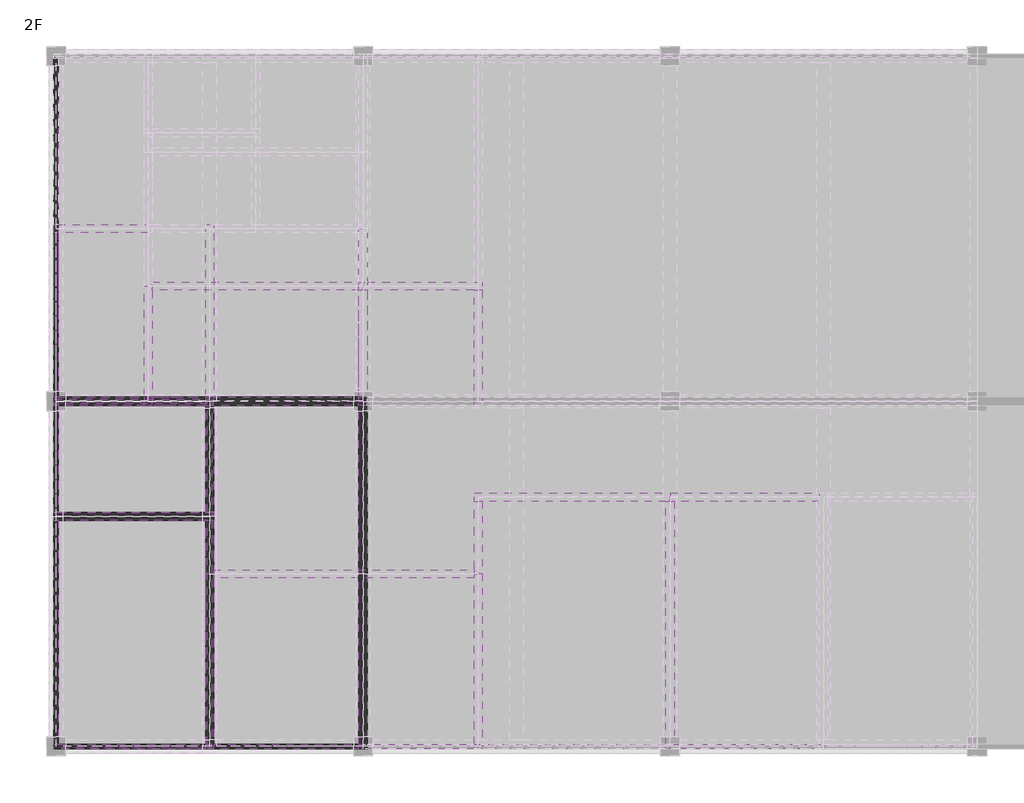
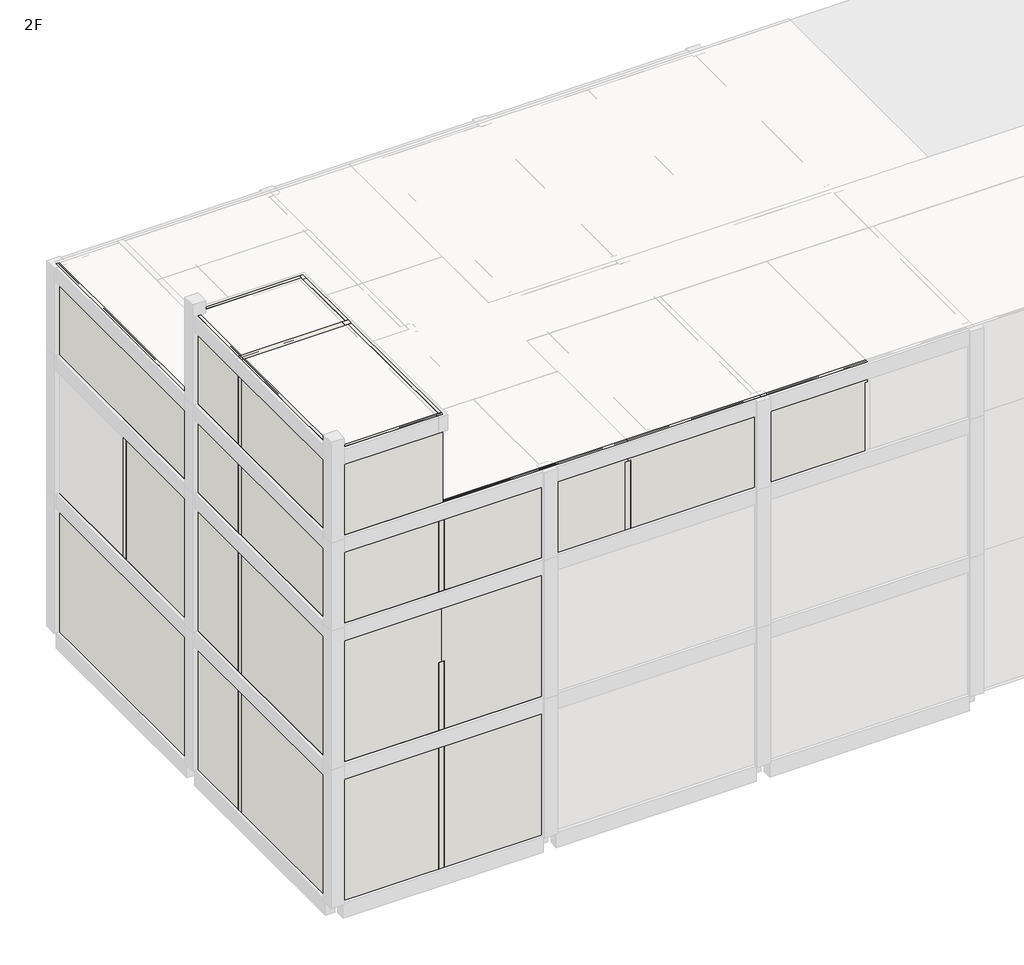
# One storey, part 1 of 7: 56 walls.
# Revit data of these elements (continued)
# Materials (continued)
#   "A04AK069-00002_Reinforced Concrete Block_THK 100-200mm": class "Concrete", colour RGB 180 180 180, transparency 0, Description = "Conc. Block", W00) Work Master Code = "A04AK069-00002", W01) Work Master_Lv1 = "Finishing Work", W02) Work Master_Lv2 = "Masonry Work", W03) Work Master_Spec.1 = "Reinforced Concrete Block", W04) Work Master_Spec.2 = "w/ All Reinf.(Lath, Steel Tie, Anchor Bar, Mortar, ETC.), Filler, Sealant, Lintel/Sill for Opening, ETC.", W05) Work Master_Spec.3 = "100mm<THK≤200mm", Cost = 0
#   "Default Wall": class "Miscellaneous", colour RGB 80 80 80, transparency 0
# Room at (79959.652, 167173.861) mm, phase "New Construction", upper offset 2700 mm, lower offset 0 mm
#   Department = "AR"
#   Base Finish = "WK3"
#   Ceiling Finish = "CL3"
#   Wall Finish = "IW5"
#   Floor Finish = "FL2"
#   Number = "4.5"
#   Name = "Office-1"
#   Interior Finish = "IW5..N/A..N/A,,WK3..N/A,,FL2..N/A,,CL3..N/A"
#   Exterior Finish = "RF1..N/A,,EW2..N/A..N/A"
# Room at (84959.652, 167173.861) mm, phase "New Construction", upper offset 3500 mm, lower offset 0 mm
#   Department = "FF"
#   Base Finish = "WK1"
#   Ceiling Finish = ""
#   Wall Finish = "IW5"
#   Floor Finish = "FL1"
#   Number = "4.6"
#   Name = "Fire Gas Room"
#   Interior Finish = "IW5..N/A..N/A,,WK1..N/A,,FL1..N/A,,N/A..N/A"
#   Exterior Finish = "RF1..N/A,,EW2..N/A..N/A"
# Room at (78709.652, 174423.861) mm, phase "New Construction", upper offset 2700 mm, lower offset 0 mm
#   Department = "AR"
#   Base Finish = "WK3"
#   Ceiling Finish = "CL3"
#   Wall Finish = "IW5"
#   Floor Finish = "FL2"
#   Number = "4.7"
#   Name = "Document Room"
#   Interior Finish = "IW5..N/A..N/A,,WK3..N/A,,FL2..N/A,,CL3..N/A"
#   Exterior Finish = "RF1..N/A,,N/A..N/A..N/A"
# Room at (58959.652, 167173.861) mm, phase "New Construction", upper offset 2700 mm, lower offset 0 mm
#   Department = "AR"
#   Base Finish = "WK3"
#   Ceiling Finish = "CL3"
#   Wall Finish = "IW5"
#   Floor Finish = "FL2"
#   Number = "4.8"
#   Name = "Storage"
#   Interior Finish = "IW5..N/A..N/A,,WK3..N/A,,FL2..N/A,,CL3..N/A"
#   Exterior Finish = "RF1..N/A,,EW1..N/A..N/A"
# Room at (52959.652, 166173.861) mm, phase "New Construction", upper offset 2700 mm, lower offset 0 mm
#   Department = "AR"
#   Base Finish = "WK3"
#   Ceiling Finish = "CL3"
#   Wall Finish = "IW5"
#   Floor Finish = "FL2"
#   Number = "4.9"
#   Name = "Break Room"
#   Interior Finish = "IW5..N/A..N/A,,WK3..N/A,,FL2..N/A,,CL3..N/A"
#   Exterior Finish = "RF1..N/A,,EW2..N/A..N/A"
# Room at (50659.652, 177673.861) mm, phase "New Construction", upper offset 2700 mm, lower offset 0 mm
#   Department = "AR"
#   Base Finish = ""
#   Ceiling Finish = "CL4"
#   Wall Finish = "IW3"
#   Floor Finish = "FL3"
#   Number = "4.10"
#   Name = "Toilet"
#   Interior Finish = "IW3..N/A..N/A,,N/A..N/A,,FL3..N/A,,CL4..N/A"
#   Exterior Finish = "RF1..N/A,,N/A..N/A..N/A"
# Room at (50659.652, 180673.861) mm, phase "New Construction", upper offset 2700 mm, lower offset 0 mm
#   Department = "AR"
#   Base Finish = ""
#   Ceiling Finish = "CL4"
#   Wall Finish = "IW3"
#   Floor Finish = "FL3"
#   Number = "4.11"
#   Name = "Shower"
#   Interior Finish = "IW3..N/A..N/A,,N/A..N/A,,FL3..N/A,,CL4..N/A"
#   Exterior Finish = "RF1..N/A,,EW2..N/A..N/A"
# Room at (61459.652, 177423.861) mm, phase "New Construction", upper offset 5500 mm, lower offset 0 mm
#   Department = "CI"
#   Base Finish = "WK1"
#   Ceiling Finish = "CL1"
#   Wall Finish = "IW5"
#   Floor Finish = "FL1"
#   Number = "2.0"
#   Name = "Electrical Room-1"
#   Interior Finish = "IW5..N/A..N/A,,WK1..N/A,,FL1..N/A,,CL1..N/A"
#   Exterior Finish = "N/A..N/A,,EW1..EW2..N/A"
# Room at (70459.652, 168423.861) mm, phase "New Construction", upper offset 5500 mm, lower offset 0 mm
#   Department = "EL"
#   Base Finish = "WK1"
#   Ceiling Finish = "CL1"
#   Wall Finish = "IW5"
#   Floor Finish = "FL1"
#   Number = "2.1"
#   Name = "Electrical Room-2"
#   Interior Finish = "IW5..N/A..N/A,,WK1..N/A,,FL1..N/A,,CL1..N/A"
#   Exterior Finish = "N/A..N/A,,EW1..EW2..N/A"
# Room at (82459.652, 177423.861) mm, phase "New Construction", upper offset 5500 mm, lower offset 0 mm
#   Department = "AR"
#   Base Finish = "WK1"
#   Ceiling Finish = "CL1"
#   Wall Finish = "IW5"
#   Floor Finish = "FL1"
#   Number = "2.2"
#   Name = "Electrical Room (GIS)"
#   Interior Finish = "IW5..N/A..N/A,,WK1..N/A,,FL1..N/A,,CL1..N/A"
#   Exterior Finish = "N/A..N/A,,EW1..EW2..N/A"
# Room at (51459.652, 168423.861) mm, phase "New Construction", upper offset 2700 mm, lower offset 0 mm
#   Department = "AR"
#   Base Finish = "WK3"
#   Ceiling Finish = "CL3"
#   Wall Finish = "IW5"
#   Floor Finish = "FL2"
#   Number = "2.3"
#   Name = "Lobby"
#   Interior Finish = "IW5..N/A..N/A,,WK3..N/A,,FL2..N/A,,CL3..N/A"
#   Exterior Finish = "N/A..N/A,,EW2..N/A..N/A"
# Room at (47459.652, 171423.861) mm, phase "New Construction", upper offset 5500 mm, lower offset 0 mm
#   Department = "PATHV2"
#   Base Finish = ""
#   Ceiling Finish = ""
#   Wall Finish = ""
#   Floor Finish = ""
#   Number = "2.4"
#   Name = "Elevator"
#   Interior Finish = "N/A..N/A..N/A,,N/A..N/A,,N/A..N/A,,N/A..N/A"
#   Exterior Finish = "N/A..N/A,,EW2..N/A..N/A"
# Room at (47459.652, 166923.861) mm, phase "New Construction", upper offset 5500 mm, lower offset 0 mm
#   Department = "PATHV1"
#   Base Finish = "WK3"
#   Ceiling Finish = "CL1"
#   Wall Finish = "IW5"
#   Floor Finish = "FL2"
#   Number = "2.5"
#   Name = "Staircase"
#   Interior Finish = "IW5..N/A..N/A,,WK3..N/A,,FL2..N/A,,CL1..N/A"
#   Exterior Finish = "N/A..N/A,,EW2..N/A..N/A"
# Room at (65459.652, 177423.861) mm, phase "New Construction", upper offset 3400 mm, lower offset 0 mm
#   Department = "CI"
#   Base Finish = ""
#   Ceiling Finish = "CL3"
#   Wall Finish = "IW5"
#   Floor Finish = "FL5"
#   Number = "3.0"
#   Name = "Central Control Room"
#   Interior Finish = "IW5..N/A..N/A,,N/A..N/A,,FL5..N/A,,CL3..N/A"
#   Exterior Finish = "N/A..N/A,,EW1..N/A..N/A"
# Room at (65459.652, 168423.861) mm, phase "New Construction", upper offset 3000 mm, lower offset 0 mm
#   Department = "CI"
#   Base Finish = ""
#   Ceiling Finish = "CL3"
#   Wall Finish = "IW5"
#   Floor Finish = "FL5"
#   Number = "3.1"
#   Name = "Electronic Room"
#   Interior Finish = "IW5..N/A..N/A,,N/A..N/A,,FL5..N/A,,CL3..N/A"
#   Exterior Finish = "N/A..N/A,,EW1..N/A..N/A"
# Room at (80959.652, 180173.861) mm, phase "New Construction", upper offset 2700 mm, lower offset 0 mm
#   Department = "AR"
#   Base Finish = ""
#   Ceiling Finish = "CL3"
#   Wall Finish = "IW5"
#   Floor Finish = "FL5"
#   Number = "3.2"
#   Name = "Computer Room"
#   Interior Finish = "IW5..N/A..N/A,,N/A..N/A,,FL5..N/A,,CL3..N/A"
#   Exterior Finish = "N/A..N/A,,EW2..N/A..N/A"
# Room at (82459.652, 168423.861) mm, phase "New Construction", upper offset 5500 mm, lower offset 0 mm
#   Department = "EL"
#   Base Finish = ""
#   Ceiling Finish = "CL3"
#   Wall Finish = "IW5"
#   Floor Finish = "FL5"
#   Number = "3.3"
#   Name = "Electrical Room -3"
#   Interior Finish = "IW5..N/A..N/A,,N/A..N/A,,FL5,,CL3..N/A"
#   Exterior Finish = "N/A..N/A,,EW2..N/A..N/A"
# Room at (80959.652, 174673.861) mm, phase "New Construction", upper offset 2700 mm, lower offset 0 mm
#   Department = "CI"
#   Base Finish = ""
#   Ceiling Finish = "CL3"
#   Wall Finish = "IW5"
#   Floor Finish = "FL5"
#   Number = "3.4"
#   Name = "Communication Room"
#   Interior Finish = "IW5..N/A..N/A,,N/A..N/A,,FL5..N/A,,CL3..N/A"
#   Exterior Finish = "N/A..N/A,,N/A..N/A..N/A"
# Room at (46659.652, 179673.861) mm, phase "New Construction", upper offset 5500 mm, lower offset 0 mm
#   Department = "PATHV3"
#   Base Finish = ""
#   Ceiling Finish = ""
#   Wall Finish = ""
#   Floor Finish = ""
#   Number = "3.5"
#   Name = "Duct Shaft"
#   Interior Finish = "N/A..N/A..N/A,,N/A..N/A,,N/A..N/A,,N/A..N/A"
#   Exterior Finish = "N/A..N/A,,EW2..N/A..N/A"
# Room at (47459.652, 175173.861) mm, phase "New Construction", upper offset 2700 mm, lower offset 0 mm
#   Department = "AR"
#   Base Finish = ""
#   Ceiling Finish = "CL4"
#   Wall Finish = "IW3"
#   Floor Finish = "FL3"
#   Number = "3.6"
#   Name = "Toilet (M)"
#   Interior Finish = "IW3..N/A..N/A,,N/A..N/A,,FL3..N/A,,CL4..N/A"
#   Exterior Finish = "N/A..N/A,,EW2..N/A..N/A"
# Room at (52059.652, 179673.861) mm, phase "New Construction", upper offset 2700 mm, lower offset 0 mm
#   Department = "AR"
#   Base Finish = ""
#   Ceiling Finish = "CL4"
#   Wall Finish = "IW3"
#   Floor Finish = "FL3"
#   Number = "3.7"
#   Name = "Toilet"
#   Interior Finish = "IW3..N/A..N/A,,N/A..N/A,,FL3..N/A,,CL4..N/A"
#   Exterior Finish = "N/A..N/A,,EW2..N/A..N/A"
# Room at (49259.652, 180923.861) mm, phase "New Construction", upper offset 2700 mm, lower offset 0 mm
#   Department = "AR"
#   Base Finish = ""
#   Ceiling Finish = "CL4"
#   Wall Finish = "IW3"
#   Floor Finish = "FL3"
#   Number = "3.8"
#   Name = "Shower"
#   Interior Finish = "IW3..N/A..N/A,,N/A..N/A,,FL3..N/A,,CL4..N/A"
#   Exterior Finish = "N/A..N/A,,EW2..N/A..N/A"
# Room at (49259.652, 178673.861) mm, phase "New Construction", upper offset 2700 mm, lower offset 0 mm
#   Department = "AR"
#   Base Finish = "WK3"
#   Ceiling Finish = "CL3"
#   Wall Finish = "IW5"
#   Floor Finish = "FL2"
#   Number = "3.9"
#   Name = "Locker(F)"
#   Interior Finish = "IW5..N/A..N/A,,WK3..N/A,,FL2..N/A,,CL3..N/A"
#   Exterior Finish = "N/A..N/A,,N/A..N/A..N/A"
# Room at (47459.652, 171423.861) mm, phase "New Construction", upper offset 5500 mm, lower offset 0 mm
#   Department = "PATHV2"
#   Base Finish = ""
#   Ceiling Finish = ""
#   Wall Finish = ""
#   Floor Finish = ""
#   Number = "3.10"
#   Name = "Elevator"
#   Interior Finish = "N/A..N/A..N/A,,N/A..N/A,,N/A..N/A,,N/A..N/A"
#   Exterior Finish = "N/A..N/A,,EW2..N/A..N/A"
# Room at (47459.652, 166923.861) mm, phase "New Construction", upper offset 2700 mm, lower offset 0 mm
#   Department = "PATHV1"
#   Base Finish = "WK3"
#   Ceiling Finish = "CL1"
#   Wall Finish = "IW5"
#   Floor Finish = "FL2"
#   Number = "3.11"
#   Name = "Staircase"
#   Interior Finish = "IW5..N/A..N/A,,WK3..N/A,,FL2..N/A,,CL1..N/A"
#   Exterior Finish = "N/A..N/A,,EW2..N/A..N/A"
# Room at (82459.652, 177423.861) mm, phase "New Construction", upper offset 2700 mm, lower offset 0 mm
#   Department = "AR"
#   Base Finish = "WK3"
#   Ceiling Finish = "CL3"
#   Wall Finish = "IW5"
#   Floor Finish = "FL2"
#   Number = "3.12"
#   Name = "Corridor"
#   Interior Finish = "IW5..N/A..N/A,,WK3..N/A,,FL2..N/A,,CL3..N/A"
#   Exterior Finish = "N/A..N/A,,EW2..N/A..N/A"
# Room at (51459.652, 170673.861) mm, phase "New Construction", upper offset 2700 mm, lower offset 0 mm
#   Department = "AR"
#   Base Finish = "WK3"
#   Ceiling Finish = "CL3"
#   Wall Finish = "IW5"
#   Floor Finish = "FL2"
#   Number = "3.13"
#   Name = "Corridor"
#   Interior Finish = "IW5..N/A..N/A,,WK3..N/A,,FL2..N/A,,CL3..N/A"
#   Exterior Finish = "N/A..N/A,,EW2..N/A..N/A"
# Room at (63459.652, 167173.861) mm, phase "New Construction", upper offset 2700 mm, lower offset 0 mm
#   Department = "AR"
#   Base Finish = "WK3"
#   Ceiling Finish = "CL3"
#   Wall Finish = "IW5"
#   Floor Finish = "FL2"
#   Number = "4.0"
#   Name = "Manager Office-1"
#   Interior Finish = "IW5..N/A..N/A,,WK3..N/A,,FL2..N/A,,CL3..N/A"
#   Exterior Finish = "RF1..N/A,,EW1..N/A..N/A"
# Room at (67459.652, 167173.861) mm, phase "New Construction", upper offset 2700 mm, lower offset 0 mm
#   Department = "AR"
#   Base Finish = "WK3"
#   Ceiling Finish = "CL3"
#   Wall Finish = "IW5"
#   Floor Finish = "FL2"
#   Number = "4.1"
#   Name = "Manager Office-2"
#   Interior Finish = "IW5..N/A..N/A,,WK3..N/A,,FL2..N/A,,CL3..N/A"
#   Exterior Finish = "RF1..N/A,,EW1..N/A..N/A"
# Room at (78709.652, 178923.861) mm, phase "New Construction", upper offset 2700 mm, lower offset 0 mm
#   Department = "AR"
#   Base Finish = "WK3"
#   Ceiling Finish = "CL3"
#   Wall Finish = "IW5"
#   Floor Finish = "FL2"
#   Number = "4.2"
#   Name = "Meeting Room-1"
#   Interior Finish = "IW5..N/A..N/A,,WK3..N/A,,FL2..N/A,,CL3..N/A"
#   Exterior Finish = "RF1..N/A,,EW1..EW2..N/A"
# Room at (73459.652, 167173.861) mm, phase "New Construction", upper offset 2700 mm, lower offset 0 mm
#   Department = "AR"
#   Base Finish = "WK3"
#   Ceiling Finish = "CL3"
#   Wall Finish = "IW5"
#   Floor Finish = "FL2"
#   Number = "4.3"
#   Name = "Meeting Room-2"
#   Interior Finish = "IW5..N/A..N/A,,WK3..N/A,,FL2..N/A,,CL3..N/A"
#   Exterior Finish = "RF1..N/A,,EW1..N/A..N/A"
# Room at (64709.652, 177423.861) mm, phase "New Construction", upper offset 2700 mm, lower offset 0 mm
#   Department = "HV"
#   Base Finish = "WK3"
#   Ceiling Finish = "CL3"
#   Wall Finish = "IW5"
#   Floor Finish = "FL2"
#   Number = "4.4"
#   Name = "Open Office"
#   Interior Finish = "IW5..N/A..N/A,,WK3..N/A,,FL2..N/A,,CL3..N/A"
#   Exterior Finish = "RF1..N/A,,EW1..N/A..N/A"
# Room at (54959.652, 178923.861) mm, phase "New Construction", upper offset 2700 mm, lower offset 0 mm
#   Department = "AR"
#   Base Finish = "WK3"
#   Ceiling Finish = "CL3"
#   Wall Finish = "IW5"
#   Floor Finish = "FL2"
#   Number = "4.12"
#   Name = "Locker(M)"
#   Interior Finish = "IW5..N/A..N/A,,WK3..N/A,,FL2..N/A,,CL3..N/A"
#   Exterior Finish = "RF1..N/A,,EW1..N/A..N/A"
# Room at (50659.652, 174423.861) mm, phase "New Construction", upper offset 2700 mm, lower offset 0 mm
#   Department = "AR"
#   Base Finish = ""
#   Ceiling Finish = "CL4"
#   Wall Finish = "IW3"
#   Floor Finish = "FL3"
#   Number = "4.13"
#   Name = "Toilet(F)"
#   Interior Finish = "IW3..N/A..N/A,,N/A..N/A,,FL3..N/A,,CL4..N/A"
#   Exterior Finish = "RF1..N/A,,N/A..N/A..N/A"
# Room at (46659.652, 177423.861) mm, phase "New Construction", upper offset 3500 mm, lower offset 0 mm
#   Department = "PATHV3"
#   Base Finish = ""
#   Ceiling Finish = ""
#   Wall Finish = ""
#   Floor Finish = ""
#   Number = "4.14"
#   Name = "Duct Shaft"
#   Interior Finish = "N/A..N/A..N/A,,N/A..N/A,,N/A..N/A,,N/A..N/A"
#   Exterior Finish = "RF1..N/A,,EW2..N/A..N/A"
# Room at (47459.652, 171423.861) mm, phase "New Construction", upper offset 3500 mm, lower offset 0 mm
#   Department = "PATHV2"
#   Base Finish = ""
#   Ceiling Finish = ""
#   Wall Finish = ""
#   Floor Finish = ""
#   Number = "4.15"
#   Name = "Elevator"
#   Interior Finish = "N/A..N/A..N/A,,N/A..N/A,,N/A..N/A,,N/A..N/A"
#   Exterior Finish = "N/A..N/A,,EW2..N/A..N/A"
# Room at (47459.652, 166923.861) mm, phase "New Construction", upper offset 3500 mm, lower offset 0 mm
#   Department = "PATHV1"
#   Base Finish = ""
#   Ceiling Finish = "CL1"
#   Wall Finish = "IW5"
#   Floor Finish = "FL2"
#   Number = "4.16"
#   Name = "Staircase"
#   Interior Finish = "IW5..N/A..N/A,,N/A..N/A,,FL2..N/A,,CL1..N/A"
#   Exterior Finish = "N/A..N/A,,EW2..N/A..N/A"
# Room at (61397.694, 171673.861) mm, phase "New Construction", upper offset 2700 mm, lower offset 0 mm
#   Department = "AR"
#   Base Finish = "WK3"
#   Ceiling Finish = "CL3"
#   Wall Finish = "IW5"
#   Floor Finish = "FL2"
#   Number = "4.17"
#   Name = "Corridor"
#   Interior Finish = "IW5..N/A..N/A,,WK3..N/A,,FL2..N/A,,CL3..N/A"
#   Exterior Finish = "RF1..N/A,,EW2..N/A..N/A"
# Room at (47459.652, 171423.861) mm, phase "New Construction", upper offset 3500 mm, lower offset 0 mm
#   Department = "PATHV2"
#   Base Finish = ""
#   Ceiling Finish = ""
#   Wall Finish = ""
#   Floor Finish = ""
#   Number = "5.0"
#   Name = "Elevator"
#   Interior Finish = "N/A..N/A..N/A,,N/A..N/A,,N/A..N/A,,N/A..N/A"
#   Exterior Finish = "RF1..N/A,,EW2..EW1..N/A"
# Room at (47459.652, 166923.861) mm, phase "New Construction", upper offset 3500 mm, lower offset 0 mm
#   Department = "PATHV1"
#   Base Finish = "WK3"
#   Ceiling Finish = "CL1"
#   Wall Finish = "IW5"
#   Floor Finish = "FL2"
#   Number = "5.1"
#   Name = "Staircase"
#   Interior Finish = "IW5..N/A..N/A,,WK3..N/A,,FL2..N/A,,CL1..N/A"
#   Exterior Finish = "RF1..N/A,,EW2..EW1..N/A"
